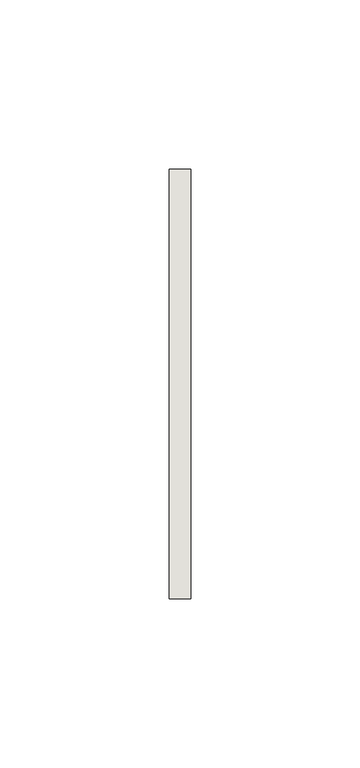
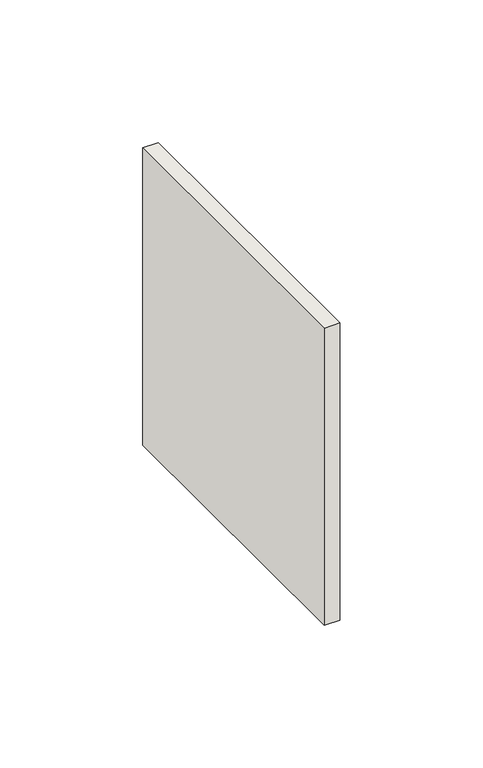
"""IFC4 building model written with IfcOpenShell, lengths in millimetres: wall geometry, TURNBUCKLET PLATE2 : TURNBUCKLET PLATE."""

from ifc_helpers import new_model, si_unit, frame, origin, place, context, project, spatial, polyline, outline, extrude, source, transform, mapped, element, save


def wall_22947521(model_context):
    return source(origin(), model_context, "Body", "SweptSolid", [
        extrude(outline(polyline([(19895.3370052, -981.5943323), (19895.3370052, -1108.5943323), (19888.9870052, -1108.5943323), (19888.9870052, -981.5943323), (19895.3370052, -981.5943323)])), frame((0.0, 0.0, 4845.2706466), z_axis=(0.0, 0.0, 1.0), x_axis=(1.0, 0.0, 0.0)), (0.0, 0.0, 1.0), 127.0),
    ])


if __name__ == "__main__":
    model = new_model("IFC4")
    model_context = context("Model", 3, world=origin())
    ifc_project = project(units=[si_unit("LENGTHUNIT", "METRE", prefix="MILLI")], contexts=[model_context])
    site = spatial("IfcSite", under=ifc_project)
    building = spatial("IfcBuilding", under=site)
    placement = place(None, origin())
    wall_shape = wall_22947521(model_context)
    element("IfcWall", 1, ObjectType="TURNBUCKLET PLATE2 : TURNBUCKLET PLATE", at=placement, inside=building, context=model_context, shape_type="MappedRepresentation", body=[
        mapped(wall_shape, transform((0.0, 0.0, 0.0), x_axis=(1.0, 0.0, 0.0), y_axis=(0.0, 1.0, 0.0), z_axis=(0.0, 0.0, 1.0))),
    ])
    save(model, "model.ifc")

# Revit data of these elements
# Element 1 (IfcWall, "TURNBUCKLET PLATE2 : TURNBUCKLET PLATE")
#   Materials on its faces: "1/4\" STEEL GUSSET PLATE - (RAW STEEL)"
# Materials
#   "1/4\" STEEL GUSSET PLATE - (RAW STEEL)": class "Metal", colour RGB 189 187 185, transparency 0, Description = "Structural steel 50ksi", Cost = 0
